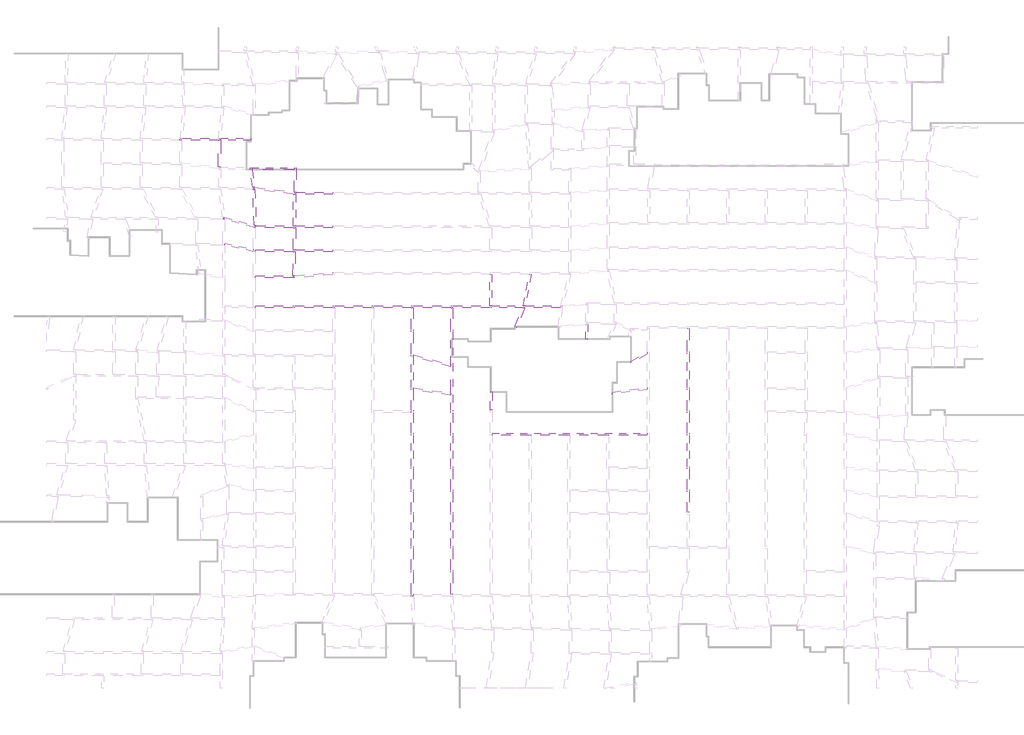
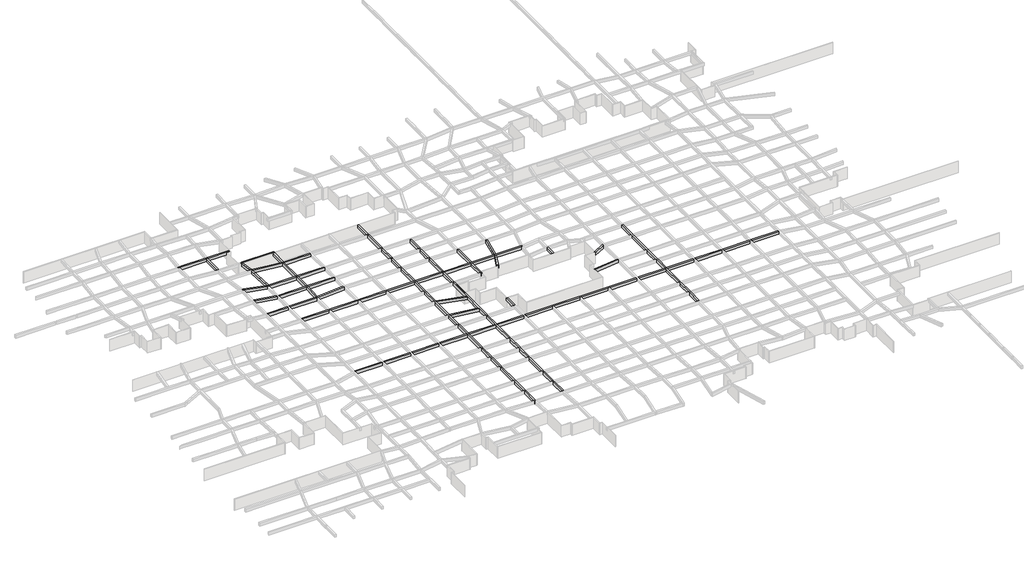
# One storey, part 28 of 45: 32 beams.
"""IFC4 building model written with IfcOpenShell, lengths in millimetres."""

import ifcopenshell
import ifcopenshell.guid

model = None  # the IFC model being written
_history = None  # IfcOwnerHistory: only IFC2X3 demands one
_inside = {}  # id of a spatial element -> (the spatial element, [elements in it])
_under = {}  # id of a project, library or spatial element -> (it, [spatial elements below it])
_declared = {}  # id of a project -> (the project, [libraries it declares])
_typed = {}  # id of a type object -> (the type object, [elements of that type])
_made_of = {}  # id of a material, layer set ... -> (it, [elements and type objects made of it])


def new_model(schema):
    """Start an empty IFC model of exactly this schema.

    Asked for "IFC4X3", IfcOpenShell would pick the latest addendum, in which some entities
    have other attributes; the version numbers below select the first issue.
    IFC2X3 requires an IfcOwnerHistory on every rooted entity: one is made here for all.
    """
    global model, _history
    if schema == "IFC4X3":
        model = ifcopenshell.file(schema_version=(4, 3, 0, 0))
    else:
        model = ifcopenshell.file(schema=schema)
    _inside.clear()
    _under.clear()
    _declared.clear()
    _typed.clear()
    _made_of.clear()
    _history = None
    if model.schema == "IFC2X3":
        org = make("IfcOrganization", Name="unknown")
        user = make(
            "IfcPersonAndOrganization",
            ThePerson=make("IfcPerson", FamilyName="unknown"),
            TheOrganization=org,
        )
        app = make(
            "IfcApplication",
            ApplicationDeveloper=org,
            Version="unknown",
            ApplicationFullName="unknown",
            ApplicationIdentifier="unknown",
        )
        _history = make(
            "IfcOwnerHistory",
            OwningUser=user,
            OwningApplication=app,
            ChangeAction="ADDED",
            CreationDate=0,
        )
    return model


def make(cls, **values):
    """One entity of the class cls with the attributes given. An attribute that is None is left unset."""
    return model.create_entity(
        cls, **{name: value for name, value in values.items() if value is not None}
    )


def rooted(cls, **values):
    """An entity with a GlobalId (a new one), such as an element, a storey or a relation."""
    return make(cls, GlobalId=ifcopenshell.guid.new(), OwnerHistory=_history, **values)


def si_unit(unit_type, name, prefix=None):
    """IfcSIUnit, for example si_unit("LENGTHUNIT", "METRE", prefix="MILLI")."""
    return make("IfcSIUnit", UnitType=unit_type, Prefix=prefix, Name=name)


def assignment(units):
    """IfcUnitAssignment: the units of a project."""
    return None if units is None else make("IfcUnitAssignment", Units=units)


def point(xyz):
    """IfcCartesianPoint."""
    return None if xyz is None else make("IfcCartesianPoint", Coordinates=xyz)


def direction(xyz):
    """IfcDirection."""
    return None if xyz is None else make("IfcDirection", DirectionRatios=xyz)


def frame(location, z_axis=None, x_axis=None):
    """IfcAxis2Placement3D, a coordinate frame: its origin and axes. An axis left out is left unset."""
    return make(
        "IfcAxis2Placement3D",
        Location=point(location),
        Axis=direction(z_axis),
        RefDirection=direction(x_axis),
    )


def origin():
    """The frame at (0, 0, 0) with its axes left unset."""
    return frame((0.0, 0.0, 0.0))


def place(relative_to, where):
    """IfcLocalPlacement: puts the frame where relative to a parent placement (None: the world)."""
    return make(
        "IfcLocalPlacement", PlacementRelTo=relative_to, RelativePlacement=where
    )


def context(
    kind, dimensions, precision=None, world=None, true_north=None, identifier=None
):
    """IfcGeometricRepresentationContext, for example the 3D "Model" context."""
    return make(
        "IfcGeometricRepresentationContext",
        ContextIdentifier=identifier,
        ContextType=kind,
        CoordinateSpaceDimension=dimensions,
        Precision=precision,
        WorldCoordinateSystem=world,
        TrueNorth=true_north,
    )


def project(units=None, contexts=None):
    """IfcProject with its units and contexts."""
    return rooted(
        "IfcProject",
        Name="project",
        RepresentationContexts=contexts,
        UnitsInContext=assignment(units),
    )


def spatial(cls, under=None, at=None, **own):
    """A site, building, storey or space (cls), placed at a placement, below another one or the project."""
    s = rooted(cls, ObjectPlacement=at, **own)
    if under is not None:
        _under.setdefault(under.id(), (under, []))[1].append(s)
    return s


def polyline(points):
    """IfcPolyline through the points."""
    return make("IfcPolyline", Points=[point(p) for p in points])


def outline(outer, holes=None, kind="AREA"):
    """IfcArbitraryClosedProfileDef: a profile drawn as a closed curve; with holes, ...WithVoids."""
    if holes is None:
        return make("IfcArbitraryClosedProfileDef", ProfileType=kind, OuterCurve=outer)
    return make(
        "IfcArbitraryProfileDefWithVoids",
        ProfileType=kind,
        OuterCurve=outer,
        InnerCurves=holes,
    )


def extrude(swept, where, along, depth):
    """IfcExtrudedAreaSolid: the profile swept, set in the frame where, extruded along a direction by depth."""
    return make(
        "IfcExtrudedAreaSolid",
        SweptArea=swept,
        Position=where,
        ExtrudedDirection=direction(along),
        Depth=depth,
    )


def faces_of(points, faces, orient=None, outer=None):
    """IfcFace entities. A face is a list of loops; a loop is a list of indices into points, from 0.

    orient and outer hold one flag for each loop. By default every Orientation is true, the
    first loop of a face is its IfcFaceOuterBound and the others are IfcFaceBound.
    """
    made = []
    for i, loops in enumerate(faces):
        bounds = []
        for j, loop in enumerate(loops):
            is_outer = j == 0 if outer is None else outer[i][j]
            bounds.append(
                make(
                    "IfcFaceOuterBound" if is_outer else "IfcFaceBound",
                    Bound=make("IfcPolyLoop", Polygon=[points[k] for k in loop]),
                    Orientation=True if orient is None else orient[i][j],
                )
            )
        made.append(make("IfcFace", Bounds=bounds))
    return made


def faceted_brep(points, faces, orient=None, outer=None, voids=None):
    """IfcFacetedBrep: a solid bounded by flat faces; with voids (closed shells), ...WithVoids."""
    shared = [point(p) for p in points]
    hull = make("IfcClosedShell", CfsFaces=faces_of(shared, faces, orient, outer))
    if voids is None:
        return make("IfcFacetedBrep", Outer=hull)
    return make(
        "IfcFacetedBrepWithVoids",
        Outer=hull,
        Voids=[
            make(cls, CfsFaces=faces_of(shared, fs, o, b)) for cls, fs, o, b in voids
        ],
    )


def shape(context_of_items, identifier, shape_type, items):
    """IfcShapeRepresentation: the items that make up one representation, for example the "Body"."""
    return make(
        "IfcShapeRepresentation",
        ContextOfItems=context_of_items,
        RepresentationIdentifier=identifier,
        RepresentationType=shape_type,
        Items=items,
    )


def made_of(thing, what):
    """Note that an element or type object is made of a material, layer set ...; save() writes the relation."""
    if what is not None:
        _made_of.setdefault(what.id(), (what, []))[1].append(thing)
    return thing


def element(
    cls,
    number,
    at=None,
    inside=None,
    cuts=None,
    type_object=None,
    material=None,
    context=None,
    identifier="Body",
    shape_type=None,
    held_by="IfcProductDefinitionShape",
    body=None,
    shapes=None,
    **own,
):
    """One element of the class cls, such as IfcWall. Its Tag is "e" and its number.

    at: its placement. inside: the storey or other place that contains it. cuts: it is an
    opening in that element (IfcRelVoidsElement). A single representation is given by context,
    identifier, shape_type and body (its items); several are given by shapes. held_by: the class
    of the entity that holds the representations. save() writes the other relations.
    """
    e = rooted(cls, Tag="e%d" % number, ObjectPlacement=at, **own)
    if body is not None:
        shapes = [shape(context, identifier, shape_type, body)]
    if shapes is not None:
        e.Representation = make(held_by, Representations=shapes)
    if inside is not None:
        _inside.setdefault(inside.id(), (inside, []))[1].append(e)
    if cuts is not None:
        rooted(
            "IfcRelVoidsElement", RelatingBuildingElement=cuts, RelatedOpeningElement=e
        )
    if type_object is not None:
        _typed.setdefault(type_object.id(), (type_object, []))[1].append(e)
    return made_of(e, material)


def aggregate(whole, parts):
    """IfcRelAggregates: a whole, such as a stair, and the parts it consists of."""
    return rooted("IfcRelAggregates", RelatingObject=whole, RelatedObjects=parts)


def save(model, path):
    """Write the relations noted so far, then the file.

    IfcRelAggregates (storeys below a building ...), IfcRelContainedInSpatialStructure (elements
    in a storey), IfcRelDefinesByType, IfcRelAssociatesMaterial and IfcRelDeclares: one each for
    every whole, place, type object, material and project.
    """
    for whole, parts in _under.values():
        aggregate(whole, parts)
    for where, things in _inside.values():
        rooted(
            "IfcRelContainedInSpatialStructure",
            RelatedElements=things,
            RelatingStructure=where,
        )
    for kind, things in _typed.values():
        rooted("IfcRelDefinesByType", RelatedObjects=things, RelatingType=kind)
    for what, things in _made_of.values():
        rooted("IfcRelAssociatesMaterial", RelatedObjects=things, RelatingMaterial=what)
    for by, libraries in _declared.values():
        rooted("IfcRelDeclares", RelatingContext=by, RelatedDefinitions=libraries)
    model.write(path)


model = new_model("IFC4")

# Units and contexts
model_context = context("Model", 3, world=origin())
ifc_project = project(units=[si_unit("LENGTHUNIT", "METRE", prefix="MILLI")], contexts=[model_context])

# Site, building, storey
site = spatial("IfcSite", under=ifc_project)
building = spatial("IfcBuilding", under=site)
storey = spatial("IfcBuildingStorey", under=building, Name="户型图", Elevation=0.0)

# Beams
placement = place(None, origin())
element("IfcBeam", 1, ObjectType="混凝土 - 矩形梁 : KL_beam", at=placement, inside=storey, context=model_context, shape_type="Brep", body=[
    faceted_brep([(-31589.1083091, 27984.5858537, 3300.0), (-31613.4317995, 28384.5858537, 3300.0), (-31838.0772004, 28384.5858537, 3300.0), (-38821.0090247, 28384.5858537, 3300.0), (-39228.4957027, 28384.5858537, 3300.0), (-45471.0209029, 28384.5858537, 3300.0), (-45871.0209029, 28384.5858537, 3300.0), (-53171.0209029, 28384.5858537, 3300.0), (-53571.0209029, 28384.5858537, 3300.0), (-60985.2176693, 28384.5858537, 3300.0), (-61385.2176693, 28384.5858537, 3300.0), (-68859.410716, 28384.5858537, 3300.0), (-69259.410716, 28384.5858537, 3300.0), (-76574.0592951, 28384.5858537, 3300.0), (-76974.0592951, 28384.5858537, 3300.0), (-84543.4535378, 28384.5858537, 3300.0), (-84943.4535378, 28384.5858537, 3300.0), (-92355.449792, 28384.5858537, 3300.0), (-92355.449792, 27984.5858537, 3300.0), (-84943.4535378, 27984.5858537, 3300.0), (-84543.4535378, 27984.5858537, 3300.0), (-76974.0592951, 27984.5858537, 3300.0), (-76574.0592951, 27984.5858537, 3300.0), (-69259.410716, 27984.5858537, 3300.0), (-68859.410716, 27984.5858537, 3300.0), (-61385.2176693, 27984.5858537, 3300.0), (-60985.2176693, 27984.5858537, 3300.0), (-53571.0209029, 27984.5858537, 3300.0), (-53171.0209029, 27984.5858537, 3300.0), (-45871.0209029, 27984.5858537, 3300.0), (-45471.0209029, 27984.5858537, 3300.0), (-39360.1406192, 27984.5858537, 3300.0), (-38928.7267221, 27984.5858537, 3300.0), (-31901.6167168, 27984.5858537, 3300.0), (-31613.4317995, 28384.5858537, 2500.0), (-31838.0772004, 28384.5858537, 2500.0), (-38821.0090247, 28384.5858537, 2500.0), (-39228.4957027, 28384.5858537, 2500.0), (-45471.0209029, 28384.5858537, 2500.0), (-45871.0209029, 28384.5858537, 2500.0), (-53171.0209029, 28384.5858537, 2500.0), (-53571.0209029, 28384.5858537, 2500.0), (-60985.2176693, 28384.5858537, 2500.0), (-61385.2176693, 28384.5858537, 2500.0), (-68859.410716, 28384.5858537, 2500.0), (-69259.410716, 28384.5858537, 2500.0), (-76574.0592951, 28384.5858537, 2500.0), (-76974.0592951, 28384.5858537, 2500.0), (-84543.4535378, 28384.5858537, 2500.0), (-84943.4535378, 28384.5858537, 2500.0), (-92355.449792, 28384.5858537, 2500.0), (-31589.1083091, 27984.5858537, 2500.0), (-31901.6167168, 27984.5858537, 2500.0), (-38928.7267221, 27984.5858537, 2500.0), (-39360.1406192, 27984.5858537, 2500.0), (-45471.0209029, 27984.5858537, 2500.0), (-45871.0209029, 27984.5858537, 2500.0), (-53171.0209029, 27984.5858537, 2500.0), (-53571.0209029, 27984.5858537, 2500.0), (-60985.2176693, 27984.5858537, 2500.0), (-61385.2176693, 27984.5858537, 2500.0), (-68859.410716, 27984.5858537, 2500.0), (-69259.410716, 27984.5858537, 2500.0), (-76574.0592951, 27984.5858537, 2500.0), (-76974.0592951, 27984.5858537, 2500.0), (-84543.4535378, 27984.5858537, 2500.0), (-84943.4535378, 27984.5858537, 2500.0), (-92355.449792, 27984.5858537, 2500.0)], [[[0, 1, 2, 3, 4, 5, 6, 7, 8, 9, 10, 11, 12, 13, 14, 15, 16, 17, 18, 19, 20, 21, 22, 23, 24, 25, 26, 27, 28, 29, 30, 31, 32, 33]], [[1, 34, 35, 36, 37, 38, 39, 40, 41, 42, 43, 44, 45, 46, 47, 48, 49, 50, 17, 16, 15, 14, 13, 12, 11, 10, 9, 8, 7, 6, 5, 4, 3, 2]], [[34, 51, 52, 53, 54, 55, 56, 57, 58, 59, 60, 61, 62, 63, 64, 65, 66, 67, 50, 49, 48, 47, 46, 45, 44, 43, 42, 41, 40, 39, 38, 37, 36, 35]], [[51, 0, 33, 32, 31, 30, 29, 28, 27, 26, 25, 24, 23, 22, 21, 20, 19, 18, 67, 66, 65, 64, 63, 62, 61, 60, 59, 58, 57, 56, 55, 54, 53, 52]], [[0, 51, 34, 1]], [[18, 17, 50, 67]]]),
])
element("IfcBeam", 2, ObjectType="混凝土 - 矩形梁 : KL_beam", at=placement, inside=storey, context=model_context, shape_type="Brep", body=[
    faceted_brep([(-60985.2176693, 55433.7567637, 3300.0), (-60985.2176693, 55433.7567637, 2500.0), (-61385.2176693, 55433.7567637, 2500.0), (-61385.2176693, 55433.7567637, 3300.0), (-60985.2176693, 50850.070339, 3300.0), (-61385.2176693, 50850.070339, 3300.0), (-61385.2176693, 50850.070339, 2500.0), (-60985.2176693, 50850.070339, 2500.0)], [[[0, 1, 2, 3]], [[4, 5, 6, 7]], [[0, 3, 5, 4]], [[3, 2, 6, 5]], [[2, 1, 7, 6]], [[1, 0, 4, 7]]]),
    faceted_brep([(-60985.2176693, -29259.522509, 3300.0), (-60985.2176693, -28866.2296815, 3300.0), (-60985.2176693, -24466.2432363, 3300.0), (-60985.2176693, -24066.2432363, 3300.0), (-60985.2176693, -19666.2432363, 3300.0), (-60985.2176693, -19266.2432363, 3300.0), (-60985.2176693, -13006.533538, 3300.0), (-60985.2176693, -12606.533538, 3300.0), (-60985.2176693, -8506.533538, 3300.0), (-60985.2176693, -8106.533538, 3300.0), (-60985.2176693, -3951.5199121, 3300.0), (-60985.2176693, -3551.5199121, 3300.0), (-60985.2176693, 2719.5822838, 3300.0), (-60985.2176693, 3119.5822838, 3300.0), (-60985.2176693, 7200.318112, 3300.0), (-60985.2176693, 7600.318112, 3300.0), (-60985.2176693, 11670.0801126, 3300.0), (-60985.2176693, 12074.0111416, 3300.0), (-60985.2176693, 18259.8013996, 3300.0), (-60985.2176693, 18673.9118717, 3300.0), (-60985.2176693, 23171.3370449, 3300.0), (-60985.2176693, 23571.3370449, 3300.0), (-60985.2176693, 27984.5858537, 3300.0), (-61385.2176693, 27984.5858537, 3300.0), (-61385.2176693, 23571.3370449, 3300.0), (-61385.2176693, 23171.3370449, 3300.0), (-61385.2176693, 18720.4464741, 3300.0), (-61385.2176693, 18320.4464741, 3300.0), (-61385.2176693, 12100.217385, 3300.0), (-61385.2176693, 11700.217385, 3300.0), (-61385.2176693, 7600.318112, 3300.0), (-61385.2176693, 7200.318112, 3300.0), (-61385.2176693, 3119.5822838, 3300.0), (-61385.2176693, 2719.5822838, 3300.0), (-61385.2176693, -3551.5199121, 3300.0), (-61385.2176693, -3951.5199121, 3300.0), (-61385.2176693, -8106.533538, 3300.0), (-61385.2176693, -8506.533538, 3300.0), (-61385.2176693, -12606.533538, 3300.0), (-61385.2176693, -13006.533538, 3300.0), (-61385.2176693, -19266.2432363, 3300.0), (-61385.2176693, -19666.2432363, 3300.0), (-61385.2176693, -24066.2432363, 3300.0), (-61385.2176693, -24466.2432363, 3300.0), (-61385.2176693, -28859.2888151, 3300.0), (-61385.2176693, -29259.522509, 3300.0), (-61385.2176693, 27984.5858537, 2500.0), (-61385.2176693, 23571.3370449, 2500.0), (-61385.2176693, 23171.3370449, 2500.0), (-61385.2176693, 18720.4464741, 2500.0), (-61385.2176693, 18320.4464741, 2500.0), (-61385.2176693, 12100.217385, 2500.0), (-61385.2176693, 11700.217385, 2500.0), (-61385.2176693, 7600.318112, 2500.0), (-61385.2176693, 7200.318112, 2500.0), (-61385.2176693, 3119.5822838, 2500.0), (-61385.2176693, 2719.5822838, 2500.0), (-61385.2176693, -3551.5199121, 2500.0), (-61385.2176693, -3951.5199121, 2500.0), (-61385.2176693, -8106.533538, 2500.0), (-61385.2176693, -8506.533538, 2500.0), (-61385.2176693, -12606.533538, 2500.0), (-61385.2176693, -13006.533538, 2500.0), (-61385.2176693, -19266.2432363, 2500.0), (-61385.2176693, -19666.2432363, 2500.0), (-61385.2176693, -24066.2432363, 2500.0), (-61385.2176693, -24466.2432363, 2500.0), (-61385.2176693, -28859.2888151, 2500.0), (-61385.2176693, -29259.522509, 2500.0), (-60985.2176693, 27984.5858537, 2500.0), (-60985.2176693, 23571.3370449, 2500.0), (-60985.2176693, 23171.3370449, 2500.0), (-60985.2176693, 18673.9118717, 2500.0), (-60985.2176693, 18259.8013996, 2500.0), (-60985.2176693, 12074.0111416, 2500.0), (-60985.2176693, 11670.0801126, 2500.0), (-60985.2176693, 7600.318112, 2500.0), (-60985.2176693, 7200.318112, 2500.0), (-60985.2176693, 3119.5822838, 2500.0), (-60985.2176693, 2719.5822838, 2500.0), (-60985.2176693, -3551.5199121, 2500.0), (-60985.2176693, -3951.5199121, 2500.0), (-60985.2176693, -8106.533538, 2500.0), (-60985.2176693, -8506.533538, 2500.0), (-60985.2176693, -12606.533538, 2500.0), (-60985.2176693, -13006.533538, 2500.0), (-60985.2176693, -19266.2432363, 2500.0), (-60985.2176693, -19666.2432363, 2500.0), (-60985.2176693, -24066.2432363, 2500.0), (-60985.2176693, -24466.2432363, 2500.0), (-60985.2176693, -28866.2296815, 2500.0), (-60985.2176693, -29259.522509, 2500.0)], [[[0, 1, 2, 3, 4, 5, 6, 7, 8, 9, 10, 11, 12, 13, 14, 15, 16, 17, 18, 19, 20, 21, 22, 23, 24, 25, 26, 27, 28, 29, 30, 31, 32, 33, 34, 35, 36, 37, 38, 39, 40, 41, 42, 43, 44, 45]], [[45, 44, 43, 42, 41, 40, 39, 38, 37, 36, 35, 34, 33, 32, 31, 30, 29, 28, 27, 26, 25, 24, 23, 46, 47, 48, 49, 50, 51, 52, 53, 54, 55, 56, 57, 58, 59, 60, 61, 62, 63, 64, 65, 66, 67, 68]], [[68, 67, 66, 65, 64, 63, 62, 61, 60, 59, 58, 57, 56, 55, 54, 53, 52, 51, 50, 49, 48, 47, 46, 69, 70, 71, 72, 73, 74, 75, 76, 77, 78, 79, 80, 81, 82, 83, 84, 85, 86, 87, 88, 89, 90, 91]], [[22, 21, 20, 19, 18, 17, 16, 15, 14, 13, 12, 11, 10, 9, 8, 7, 6, 5, 4, 3, 2, 1, 0, 91, 90, 89, 88, 87, 86, 85, 84, 83, 82, 81, 80, 79, 78, 77, 76, 75, 74, 73, 72, 71, 70, 69]], [[23, 22, 69, 46]], [[0, 45, 68, 91]]]),
    faceted_brep([(-60985.2176693, 28384.5858537, 3300.0), (-61385.2176693, 28384.5858537, 3300.0), (-61385.2176693, 28384.5858537, 2500.0), (-60985.2176693, 28384.5858537, 2500.0), (-60985.2176693, 34571.3370449, 3300.0), (-61385.2176693, 34571.3370449, 3300.0), (-61385.2176693, 34571.3370449, 2500.0), (-60985.2176693, 34571.3370449, 2500.0)], [[[0, 1, 2, 3]], [[1, 0, 4, 5]], [[2, 1, 5, 6]], [[3, 2, 6, 7]], [[0, 3, 7, 4]], [[5, 4, 7, 6]]]),
    faceted_brep([(-60985.2176693, 34971.3370449, 3300.0), (-61385.2176693, 34971.3370449, 3300.0), (-61385.2176693, 34971.3370449, 2500.0), (-60985.2176693, 34971.3370449, 2500.0), (-60985.2176693, 39070.5101546, 3300.0), (-61385.2176693, 39070.5101546, 3300.0), (-61385.2176693, 39070.5101546, 2500.0), (-60985.2176693, 39070.5101546, 2500.0)], [[[0, 1, 2, 3]], [[1, 0, 4, 5]], [[2, 1, 5, 6]], [[3, 2, 6, 7]], [[0, 3, 7, 4]], [[5, 4, 7, 6]]]),
    faceted_brep([(-60985.2176693, 39470.5101546, 3300.0), (-61385.2176693, 39470.5101546, 3300.0), (-61385.2176693, 39470.5101546, 2500.0), (-60985.2176693, 39470.5101546, 2500.0), (-60985.2176693, 43842.2010773, 3300.0), (-61385.2176693, 43842.2010773, 3300.0), (-61385.2176693, 43842.2010773, 2500.0), (-60985.2176693, 43842.2010773, 2500.0)], [[[0, 1, 2, 3]], [[1, 0, 4, 5]], [[2, 1, 5, 6]], [[3, 2, 6, 7]], [[0, 3, 7, 4]], [[5, 4, 7, 6]]]),
    faceted_brep([(-60985.2176693, 44242.2010773, 3300.0), (-61385.2176693, 44242.2010773, 3300.0), (-61385.2176693, 44242.2010773, 2500.0), (-60985.2176693, 44242.2010773, 2500.0), (-60985.2176693, 50450.070339, 3300.0), (-61385.2176693, 50450.070339, 3300.0), (-61385.2176693, 50450.070339, 2500.0), (-60985.2176693, 50450.070339, 2500.0)], [[[0, 1, 2, 3]], [[1, 0, 4, 5]], [[2, 1, 5, 6]], [[3, 2, 6, 7]], [[0, 3, 7, 4]], [[5, 4, 7, 6]]]),
])
element("IfcBeam", 3, ObjectType="混凝土 - 矩形梁 : KL_beam", at=placement, inside=storey, context=model_context, shape_type="Brep", body=[
    faceted_brep([(-53171.0209029, 43842.2010773, 3300.0), (-53571.0209029, 43842.2010773, 3300.0), (-53571.0209029, 39470.5101546, 3300.0), (-53171.0209029, 39470.5101546, 3300.0), (-53571.0209029, 43842.2010773, 2500.0), (-53571.0209029, 39470.5101546, 2500.0), (-53171.0209029, 43842.2010773, 2500.0), (-53171.0209029, 39470.5101546, 2500.0)], [[[0, 1, 2, 3]], [[1, 4, 5, 2]], [[4, 6, 7, 5]], [[6, 0, 3, 7]], [[1, 0, 6, 4]], [[3, 2, 5, 7]]]),
    faceted_brep([(-53171.0209029, 28384.5858537, 3300.0), (-53571.0209029, 28384.5858537, 3300.0), (-53571.0209029, 28384.5858537, 2500.0), (-53171.0209029, 28384.5858537, 2500.0), (-53571.0209029, 34571.3370449, 3300.0), (-53171.0209029, 34571.3370449, 3300.0), (-53171.0209029, 34571.3370449, 2500.0), (-53571.0209029, 34571.3370449, 2500.0)], [[[0, 1, 2, 3]], [[4, 5, 6, 7]], [[1, 0, 5, 4]], [[2, 1, 4, 7]], [[3, 2, 7, 6]], [[0, 3, 6, 5]]]),
    faceted_brep([(-53571.0209029, 27984.5858537, 3300.0), (-53171.0209029, 27984.5858537, 3300.0), (-53171.0209029, 27984.5858537, 2500.0), (-53571.0209029, 27984.5858537, 2500.0), (-53571.0209029, 23571.3370449, 3300.0), (-53571.0209029, 23171.3370449, 3300.0), (-53571.0209029, 16687.2838357, 3300.0), (-53571.0209029, 16273.1733635, 3300.0), (-53571.0209029, 11032.0137394, 3300.0), (-53571.0209029, 10628.0827104, 3300.0), (-53571.0209029, 7600.318112, 3300.0), (-53571.0209029, 7200.318112, 3300.0), (-53571.0209029, 3119.5822838, 3300.0), (-53571.0209029, 2719.5822838, 3300.0), (-53571.0209029, -3551.5199121, 3300.0), (-53571.0209029, -3951.5199121, 3300.0), (-53571.0209029, -8106.533538, 3300.0), (-53571.0209029, -8506.533538, 3300.0), (-53571.0209029, -12606.533538, 3300.0), (-53571.0209029, -13006.533538, 3300.0), (-53571.0209029, -19266.2432363, 3300.0), (-53571.0209029, -19666.2432363, 3300.0), (-53571.0209029, -24066.2432363, 3300.0), (-53571.0209029, -24466.2432363, 3300.0), (-53571.0209029, -28866.2296815, 3300.0), (-53171.0209029, -28866.2296815, 3300.0), (-53171.0209029, -24466.2432363, 3300.0), (-53171.0209029, -24066.2432363, 3300.0), (-53171.0209029, -19666.2432363, 3300.0), (-53171.0209029, -19266.2432363, 3300.0), (-53171.0209029, -13006.533538, 3300.0), (-53171.0209029, -12606.533538, 3300.0), (-53171.0209029, -8506.533538, 3300.0), (-53171.0209029, -8106.533538, 3300.0), (-53171.0209029, -3951.5199121, 3300.0), (-53171.0209029, -3551.5199121, 3300.0), (-53171.0209029, 2719.5822838, 3300.0), (-53171.0209029, 3119.5822838, 3300.0), (-53171.0209029, 7200.318112, 3300.0), (-53171.0209029, 7600.318112, 3300.0), (-53171.0209029, 23171.3370449, 3300.0), (-53171.0209029, 23571.3370449, 3300.0), (-53571.0209029, 23571.3370449, 2500.0), (-53571.0209029, 23171.3370449, 2500.0), (-53571.0209029, 16687.2838357, 2500.0), (-53571.0209029, 16273.1733635, 2500.0), (-53571.0209029, 11032.0137394, 2500.0), (-53571.0209029, 10628.0827104, 2500.0), (-53571.0209029, 7600.318112, 2500.0), (-53571.0209029, 7200.318112, 2500.0), (-53571.0209029, 3119.5822838, 2500.0), (-53571.0209029, 2719.5822838, 2500.0), (-53571.0209029, -3551.5199121, 2500.0), (-53571.0209029, -3951.5199121, 2500.0), (-53571.0209029, -8106.533538, 2500.0), (-53571.0209029, -8506.533538, 2500.0), (-53571.0209029, -12606.533538, 2500.0), (-53571.0209029, -13006.533538, 2500.0), (-53571.0209029, -19266.2432363, 2500.0), (-53571.0209029, -19666.2432363, 2500.0), (-53571.0209029, -24066.2432363, 2500.0), (-53571.0209029, -24466.2432363, 2500.0), (-53571.0209029, -28866.2296815, 2500.0), (-53171.0209029, 23571.3370449, 2500.0), (-53171.0209029, 23171.3370449, 2500.0), (-53171.0209029, 7600.318112, 2500.0), (-53171.0209029, 7200.318112, 2500.0), (-53171.0209029, 3119.5822838, 2500.0), (-53171.0209029, 2719.5822838, 2500.0), (-53171.0209029, -3551.5199121, 2500.0), (-53171.0209029, -3951.5199121, 2500.0), (-53171.0209029, -8106.533538, 2500.0), (-53171.0209029, -8506.533538, 2500.0), (-53171.0209029, -12606.533538, 2500.0), (-53171.0209029, -13006.533538, 2500.0), (-53171.0209029, -19266.2432363, 2500.0), (-53171.0209029, -19666.2432363, 2500.0), (-53171.0209029, -24066.2432363, 2500.0), (-53171.0209029, -24466.2432363, 2500.0), (-53171.0209029, -28866.2296815, 2500.0)], [[[0, 1, 2, 3]], [[1, 0, 4, 5, 6, 7, 8, 9, 10, 11, 12, 13, 14, 15, 16, 17, 18, 19, 20, 21, 22, 23, 24, 25, 26, 27, 28, 29, 30, 31, 32, 33, 34, 35, 36, 37, 38, 39, 40, 41]], [[0, 3, 42, 43, 44, 45, 46, 47, 48, 49, 50, 51, 52, 53, 54, 55, 56, 57, 58, 59, 60, 61, 62, 24, 23, 22, 21, 20, 19, 18, 17, 16, 15, 14, 13, 12, 11, 10, 9, 8, 7, 6, 5, 4]], [[3, 2, 63, 64, 65, 66, 67, 68, 69, 70, 71, 72, 73, 74, 75, 76, 77, 78, 79, 62, 61, 60, 59, 58, 57, 56, 55, 54, 53, 52, 51, 50, 49, 48, 47, 46, 45, 44, 43, 42]], [[2, 1, 41, 40, 39, 38, 37, 36, 35, 34, 33, 32, 31, 30, 29, 28, 27, 26, 25, 79, 78, 77, 76, 75, 74, 73, 72, 71, 70, 69, 68, 67, 66, 65, 64, 63]], [[25, 24, 62, 79]]]),
    faceted_brep([(-53171.0209029, 34971.3370449, 3300.0), (-53571.0209029, 34971.3370449, 3300.0), (-53571.0209029, 34971.3370449, 2500.0), (-53171.0209029, 34971.3370449, 2500.0), (-53571.0209029, 39070.5101546, 3300.0), (-53171.0209029, 39070.5101546, 3300.0), (-53171.0209029, 39070.5101546, 2500.0), (-53571.0209029, 39070.5101546, 2500.0)], [[[0, 1, 2, 3]], [[4, 5, 6, 7]], [[1, 0, 5, 4]], [[2, 1, 4, 7]], [[3, 2, 7, 6]], [[0, 3, 6, 5]]]),
])
element("IfcBeam", 4, ObjectType="混凝土 - 矩形梁 : KL_beam", at=placement, inside=storey, context=model_context, shape_type="Brep", body=[
    faceted_brep([(-6328.2347705, 23868.127427, 3300.0), (-6728.2347705, 23868.127427, 3300.0), (-6728.2347705, 19231.9876735, 3300.0), (-6728.2347705, 18831.9876735, 3300.0), (-6728.2347705, 12131.9876735, 3300.0), (-6728.2347705, 11731.9876735, 3300.0), (-6728.2347705, 7519.5822838, 3300.0), (-6728.2347705, 7119.5822838, 3300.0), (-6728.2347705, 3119.5822838, 3300.0), (-6728.2347705, 2719.5822838, 3300.0), (-6728.2347705, -3551.5199121, 3300.0), (-6728.2347705, -3951.5199121, 3300.0), (-6728.2347705, -8106.533538, 3300.0), (-6728.2347705, -8506.533538, 3300.0), (-6728.2347705, -12606.533538, 3300.0), (-6328.2347705, -12606.533538, 3300.0), (-6328.2347705, -8506.533538, 3300.0), (-6328.2347705, -8106.533538, 3300.0), (-6328.2347705, -3951.5199121, 3300.0), (-6328.2347705, -3551.5199121, 3300.0), (-6328.2347705, 2719.5822838, 3300.0), (-6328.2347705, 3119.5822838, 3300.0), (-6328.2347705, 7119.5822838, 3300.0), (-6328.2347705, 7519.5822838, 3300.0), (-6328.2347705, 11731.9876735, 3300.0), (-6328.2347705, 12131.9876735, 3300.0), (-6328.2347705, 18831.9876735, 3300.0), (-6328.2347705, 19231.9876735, 3300.0), (-6728.2347705, 23868.127427, 2500.0), (-6728.2347705, 19231.9876735, 2500.0), (-6728.2347705, 18831.9876735, 2500.0), (-6728.2347705, 12131.9876735, 2500.0), (-6728.2347705, 11731.9876735, 2500.0), (-6728.2347705, 7519.5822838, 2500.0), (-6728.2347705, 7119.5822838, 2500.0), (-6728.2347705, 3119.5822838, 2500.0), (-6728.2347705, 2719.5822838, 2500.0), (-6728.2347705, -3551.5199121, 2500.0), (-6728.2347705, -3951.5199121, 2500.0), (-6728.2347705, -8106.533538, 2500.0), (-6728.2347705, -8506.533538, 2500.0), (-6728.2347705, -12606.533538, 2500.0), (-6328.2347705, 23868.127427, 2500.0), (-6328.2347705, 19231.9876735, 2500.0), (-6328.2347705, 18831.9876735, 2500.0), (-6328.2347705, 12131.9876735, 2500.0), (-6328.2347705, 11731.9876735, 2500.0), (-6328.2347705, 7519.5822838, 2500.0), (-6328.2347705, 7119.5822838, 2500.0), (-6328.2347705, 3119.5822838, 2500.0), (-6328.2347705, 2719.5822838, 2500.0), (-6328.2347705, -3551.5199121, 2500.0), (-6328.2347705, -3951.5199121, 2500.0), (-6328.2347705, -8106.533538, 2500.0), (-6328.2347705, -8506.533538, 2500.0), (-6328.2347705, -12606.533538, 2500.0)], [[[0, 1, 2, 3, 4, 5, 6, 7, 8, 9, 10, 11, 12, 13, 14, 15, 16, 17, 18, 19, 20, 21, 22, 23, 24, 25, 26, 27]], [[1, 28, 29, 30, 31, 32, 33, 34, 35, 36, 37, 38, 39, 40, 41, 14, 13, 12, 11, 10, 9, 8, 7, 6, 5, 4, 3, 2]], [[28, 42, 43, 44, 45, 46, 47, 48, 49, 50, 51, 52, 53, 54, 55, 41, 40, 39, 38, 37, 36, 35, 34, 33, 32, 31, 30, 29]], [[42, 0, 27, 26, 25, 24, 23, 22, 21, 20, 19, 18, 17, 16, 15, 55, 54, 53, 52, 51, 50, 49, 48, 47, 46, 45, 44, 43]], [[1, 0, 42, 28]], [[15, 14, 41, 55]]]),
])
element("IfcBeam", 5, ObjectType="混凝土 - 矩形梁 : KL_beam", at=placement, inside=storey, context=model_context, shape_type="SweptSolid", body=[
    extrude(outline(polyline([(-38821.0090247, 28384.5858537), (-39228.4957027, 28384.5858537), (-38025.9130936, 34571.3370449), (-37618.4264156, 34571.3370449), (-38821.0090247, 28384.5858537)])), frame((0.0, 0.0, 2500.0), z_axis=(0.0, 0.0, 1.0), x_axis=(1.0, 0.0, 0.0)), (0.0, 0.0, 1.0), 800.0),
])
element("IfcBeam", 6, ObjectType="混凝土 - 矩形梁 : KL_beam", at=placement, inside=storey, context=model_context, shape_type="Brep", body=[
    faceted_brep([(-45471.0209029, 34571.3370449, 3300.0), (-45871.0209029, 34571.3370449, 3300.0), (-45871.0209029, 28384.5858537, 3300.0), (-45471.0209029, 28384.5858537, 3300.0), (-45871.0209029, 34571.3370449, 2500.0), (-45871.0209029, 28384.5858537, 2500.0), (-45471.0209029, 34571.3370449, 2500.0), (-45471.0209029, 28384.5858537, 2500.0)], [[[0, 1, 2, 3]], [[1, 4, 5, 2]], [[4, 6, 7, 5]], [[6, 0, 3, 7]], [[1, 0, 6, 4]], [[3, 2, 5, 7]]]),
    faceted_brep([(-45871.0209029, 27984.5858537, 3300.0), (-45471.0209029, 27984.5858537, 3300.0), (-45471.0209029, 27984.5858537, 2500.0), (-45871.0209029, 27984.5858537, 2500.0), (-45871.0209029, 23171.3370449, 3300.0), (-45471.0209029, 23171.3370449, 3300.0), (-45871.0209029, 23571.3370449, 3300.0), (-45871.0209029, 23171.3370449, 2500.0), (-45871.0209029, 23571.3370449, 2500.0), (-45471.0209029, 23171.3370449, 2500.0)], [[[0, 1, 2, 3]], [[4, 5, 1, 0, 6]], [[7, 4, 6, 0, 3, 8]], [[9, 7, 8, 3, 2]], [[5, 9, 2, 1]], [[5, 4, 7, 9]]]),
])
element("IfcBeam", 7, ObjectType="混凝土 - 矩形梁 : KL_beam", at=placement, inside=storey, context=model_context, shape_type="Brep", body=[
    faceted_brep([(-99250.9559359, 61170.3096597, 3300.0), (-99209.2278595, 61570.3096597, 3300.0), (-99611.3985103, 61570.3096597, 3300.0), (-106787.9351309, 61570.3096597, 3300.0), (-107189.4630659, 61570.3096597, 3300.0), (-107354.1744669, 61570.3096597, 3300.0), (-107354.1744669, 61170.3096597, 3300.0), (-106954.1744669, 61170.3096597, 3300.0), (-99631.1820439, 61170.3096597, 3300.0), (-99250.9559359, 61170.3096597, 2500.0), (-107354.1744669, 61170.3096597, 2500.0), (-106954.1744669, 61170.3096597, 2500.0), (-99631.1820439, 61170.3096597, 2500.0), (-99209.2278595, 61570.3096597, 2500.0), (-107354.1744669, 61570.3096597, 2500.0), (-107189.4630659, 61570.3096597, 2500.0), (-106787.9351309, 61570.3096597, 2500.0), (-99611.3985103, 61570.3096597, 2500.0)], [[[0, 1, 2, 3, 4, 5, 6, 7, 8]], [[9, 0, 8, 7, 6, 10, 11, 12]], [[13, 9, 12, 11, 10, 14, 15, 16, 17]], [[1, 13, 17, 16, 15, 14, 5, 4, 3, 2]], [[1, 0, 9, 13]], [[6, 5, 14, 10]]]),
])
element("IfcBeam", 8, ObjectType="混凝土 - 矩形梁 : KL_beam", at=placement, inside=storey, context=model_context, shape_type="Brep", body=[
    faceted_brep([(-93231.1772231, 61570.3096597, 3300.0), (-93231.1772231, 61170.3096597, 3300.0), (-93231.1772231, 61170.3096597, 2500.0), (-93231.1772231, 61570.3096597, 2500.0), (-99209.2278595, 61570.3096597, 3300.0), (-99250.9559359, 61170.3096597, 3300.0), (-99231.1820439, 61170.3096597, 3300.0), (-99250.9559359, 61170.3096597, 2500.0), (-99231.1820439, 61170.3096597, 2500.0), (-99209.2278595, 61570.3096597, 2500.0)], [[[0, 1, 2, 3]], [[1, 0, 4, 5, 6]], [[2, 1, 6, 5, 7, 8]], [[3, 2, 8, 7, 9]], [[0, 3, 9, 4]], [[5, 4, 9, 7]]]),
])
element("IfcBeam", 9, ObjectType="混凝土 - 矩形梁 : KL_beam", at=placement, inside=storey, context=model_context, shape_type="Brep", body=[
    faceted_brep([(-84245.4455357, 50827.038832, 3300.0), (-84645.4455357, 50876.1526564, 3300.0), (-92452.2931975, 51834.7130186, 3300.0), (-92616.9469361, 51854.9299556, 3300.0), (-92641.4119842, 51454.9299556, 3300.0), (-92421.2676267, 51427.8996273, 3300.0), (-84764.7545436, 50487.7980304, 3300.0), (-84364.7545436, 50438.684206, 3300.0), (-84294.1932731, 50430.0203714, 3300.0), (-84289.9298602, 50464.7430833, 3300.0), (-92641.4119842, 51454.9299556, 2500.0), (-92421.2676267, 51427.8996273, 2500.0), (-84764.7545436, 50487.7980304, 2500.0), (-84364.7545436, 50438.684206, 2500.0), (-84294.1932731, 50430.0203714, 2500.0), (-92616.9469361, 51854.9299556, 2500.0), (-92452.2931975, 51834.7130186, 2500.0), (-84645.4455357, 50876.1526564, 2500.0), (-84245.4455357, 50827.038832, 2500.0), (-84289.9298602, 50464.7430833, 2500.0)], [[[0, 1, 2, 3, 4, 5, 6, 7, 8, 9]], [[8, 7, 6, 5, 4, 10, 11, 12, 13, 14]], [[14, 13, 12, 11, 10, 15, 16, 17, 18, 19]], [[3, 2, 1, 0, 18, 17, 16, 15]], [[3, 15, 10, 4]], [[0, 9, 8, 14, 19, 18]]]),
])
element("IfcBeam", 10, ObjectType="混凝土 - 矩形梁 : KL_beam", at=placement, inside=storey, context=model_context, shape_type="Brep", body=[
    faceted_brep([(-92452.2931975, 51834.7130186, 3300.0), (-92946.3477439, 55350.0937791, 3300.0), (-93002.5640778, 55750.0937791, 3300.0), (-93021.5786579, 55747.4214542, 3300.0), (-93398.6713053, 55694.4245387, 3300.0), (-93350.7020276, 55353.1053927, 3300.0), (-92859.0655317, 51854.9299556, 3300.0), (-92616.9469361, 51854.9299556, 3300.0), (-92452.2931975, 51834.7130186, 2500.0), (-92946.3477439, 55350.0937791, 2500.0), (-93002.5640778, 55750.0937791, 2500.0), (-92616.9469361, 51854.9299556, 2500.0), (-92859.0655317, 51854.9299556, 2500.0), (-93350.7020276, 55353.1053927, 2500.0), (-93398.6713053, 55694.4245387, 2500.0), (-93021.5786579, 55747.4214542, 2500.0)], [[[0, 1, 2, 3, 4, 5, 6, 7]], [[2, 1, 0, 8, 9, 10]], [[10, 9, 8, 11, 12, 13, 14, 15]], [[4, 14, 13, 12, 6, 5]], [[0, 7, 11, 8]], [[7, 6, 12, 11]], [[4, 3, 2, 10, 15, 14]]]),
])
element("IfcBeam", 11, ObjectType="混凝土 - 矩形梁 : KL_beam", at=placement, inside=storey, context=model_context, shape_type="Brep", body=[
    faceted_brep([(-84245.4455357, 55750.0937791, 3300.0), (-84645.4455357, 55750.0937791, 3300.0), (-84645.4455357, 55350.0937791, 3300.0), (-84645.4455357, 50876.1526564, 3300.0), (-84245.4455357, 50827.038832, 3300.0), (-84245.4455357, 50864.7430833, 3300.0), (-84245.4455357, 55750.0937791, 2500.0), (-84245.4455357, 50827.038832, 2500.0), (-84245.4455357, 50864.7430833, 2500.0), (-84645.4455357, 55750.0937791, 2500.0), (-84645.4455357, 50876.1526564, 2500.0), (-84645.4455357, 55350.0937791, 2500.0)], [[[0, 1, 2, 3, 4, 5]], [[6, 0, 5, 4, 7, 8]], [[9, 6, 8, 7, 10, 11]], [[1, 9, 11, 10, 3, 2]], [[4, 3, 10, 7]], [[1, 0, 6, 9]]]),
])
element("IfcBeam", 12, ObjectType="混凝土 - 矩形梁 : KL_beam", at=placement, inside=storey, context=model_context, shape_type="SweptSolid", body=[
    extrude(outline(polyline([(-92946.3477439, 55350.0937791), (-93002.5640778, 55750.0937791), (-84645.4455357, 55750.0937791), (-84645.4455357, 55350.0937791), (-92946.3477439, 55350.0937791)])), frame((0.0, 0.0, 2500.0), z_axis=(0.0, 0.0, 1.0), x_axis=(1.0, 0.0, 0.0)), (0.0, 0.0, 1.0), 800.0),
])
element("IfcBeam", 13, ObjectType="混凝土 - 矩形梁 : KL_beam", at=placement, inside=storey, context=model_context, shape_type="Brep", body=[
    faceted_brep([(-99631.1820439, 55886.0592094, 3300.0), (-99363.3334842, 55858.1171964, 3300.0), (-99231.1820439, 55855.8104845, 3300.0), (-99231.1820439, 61170.3096597, 3300.0), (-99250.9559359, 61170.3096597, 3300.0), (-99631.1820439, 61170.3096597, 3300.0), (-99631.1820439, 55886.0592094, 2500.0), (-99631.1820439, 61170.3096597, 2500.0), (-99363.3334842, 55858.1171964, 2500.0), (-99250.9559359, 61170.3096597, 2500.0), (-99231.1820439, 61170.3096597, 2500.0), (-99231.1820439, 55855.8104845, 2500.0)], [[[0, 1, 2, 3, 4, 5]], [[6, 0, 5, 7]], [[8, 6, 7, 9, 10, 11]], [[10, 3, 2, 11]], [[1, 0, 6, 8]], [[7, 5, 4, 3, 10, 9]], [[2, 1, 8, 11]]]),
])
element("IfcBeam", 14, ObjectType="混凝土 - 矩形梁 : KL_beam", at=placement, inside=storey, context=model_context, shape_type="Brep", body=[
    faceted_brep([(-92329.1192925, 44242.2010773, 3300.0), (-92564.8658583, 44305.3691792, 3300.0), (-98452.964117, 45883.0803526, 3300.0), (-98608.2051581, 45924.6770642, 3300.0), (-98660.8661571, 45524.6770642, 3300.0), (-98434.5356576, 45464.0319896, 3300.0), (-92755.449792, 43942.3255182, 3300.0), (-92381.7802915, 43842.2010773, 3300.0), (-98660.8661571, 45524.6770642, 2500.0), (-98434.5356576, 45464.0319896, 2500.0), (-92755.449792, 43942.3255182, 2500.0), (-92381.7802915, 43842.2010773, 2500.0), (-98608.2051581, 45924.6770642, 2500.0), (-98452.964117, 45883.0803526, 2500.0), (-92564.8658583, 44305.3691792, 2500.0), (-92329.1192925, 44242.2010773, 2500.0)], [[[0, 1, 2, 3, 4, 5, 6, 7]], [[7, 6, 5, 4, 8, 9, 10, 11]], [[11, 10, 9, 8, 12, 13, 14, 15]], [[3, 2, 1, 0, 15, 14, 13, 12]], [[3, 12, 8, 4]], [[0, 7, 11, 15]]]),
])
element("IfcBeam", 15, ObjectType="混凝土 - 矩形梁 : KL_beam", at=placement, inside=storey, context=model_context, shape_type="Brep", body=[
    faceted_brep([(-92329.1192925, 44242.2010773, 3300.0), (-92381.7802915, 43842.2010773, 3300.0), (-92355.449792, 43842.2010773, 3300.0), (-84764.7545436, 43842.2010773, 3300.0), (-84364.7545436, 43842.2010773, 3300.0), (-76974.0592951, 43842.2010773, 3300.0), (-76974.0592951, 44242.2010773, 3300.0), (-84364.7545436, 44242.2010773, 3300.0), (-84764.7545436, 44242.2010773, 3300.0), (-92162.3299648, 44242.2010773, 3300.0), (-92329.1192925, 44242.2010773, 2500.0), (-76974.0592951, 44242.2010773, 2500.0), (-84364.7545436, 44242.2010773, 2500.0), (-84764.7545436, 44242.2010773, 2500.0), (-92162.3299648, 44242.2010773, 2500.0), (-92381.7802915, 43842.2010773, 2500.0), (-76974.0592951, 43842.2010773, 2500.0), (-84364.7545436, 43842.2010773, 2500.0), (-84764.7545436, 43842.2010773, 2500.0), (-92355.449792, 43842.2010773, 2500.0)], [[[0, 1, 2, 3, 4, 5, 6, 7, 8, 9]], [[10, 0, 9, 8, 7, 6, 11, 12, 13, 14]], [[15, 10, 14, 13, 12, 11, 16, 17, 18, 19]], [[1, 15, 19, 18, 17, 16, 5, 4, 3, 2]], [[1, 0, 10, 15]], [[6, 5, 16, 11]]]),
])
element("IfcBeam", 16, ObjectType="混凝土 - 矩形梁 : KL_beam", at=placement, inside=storey, context=model_context, shape_type="SweptSolid", body=[
    extrude(outline(polyline([(-92162.3299648, 44242.2010773), (-92329.1192925, 44242.2010773), (-92564.8658583, 44305.3691792), (-92822.5012905, 51454.9299556), (-92641.4119842, 51454.9299556), (-92421.2676267, 51427.8996273), (-92162.3299648, 44242.2010773)])), frame((0.0, 0.0, 2500.0), z_axis=(0.0, 0.0, 1.0), x_axis=(1.0, 0.0, 0.0)), (0.0, 0.0, 1.0), 800.0),
])
element("IfcBeam", 17, ObjectType="混凝土 - 矩形梁 : KL_beam", at=placement, inside=storey, context=model_context, shape_type="Brep", body=[
    faceted_brep([(-84364.7545436, 50438.684206, 3300.0), (-84645.4455357, 50473.1487262, 3300.0), (-84764.7545436, 50487.7980304, 3300.0), (-84764.7545436, 44242.2010773, 3300.0), (-84364.7545436, 44242.2010773, 3300.0), (-84364.7545436, 50438.684206, 2500.0), (-84364.7545436, 44242.2010773, 2500.0), (-84764.7545436, 50487.7980304, 2500.0), (-84645.4455357, 50473.1487262, 2500.0), (-84764.7545436, 44242.2010773, 2500.0)], [[[0, 1, 2, 3, 4]], [[5, 0, 4, 6]], [[7, 8, 5, 6, 9]], [[2, 7, 9, 3]], [[0, 5, 8, 7, 2, 1]], [[4, 3, 9, 6]]]),
])
element("IfcBeam", 18, ObjectType="混凝土 - 矩形梁 : KL_beam", at=placement, inside=storey, context=model_context, shape_type="SweptSolid", body=[
    extrude(outline(polyline([(-60985.2176693, 11670.0801126), (-60985.2176693, 12074.0111416), (-53571.0209029, 11032.0137394), (-53571.0209029, 10628.0827104), (-60985.2176693, 11670.0801126)])), frame((0.0, 0.0, 2500.0), z_axis=(0.0, 0.0, 1.0), x_axis=(1.0, 0.0, 0.0)), (0.0, 0.0, 1.0), 800.0),
])
element("IfcBeam", 19, ObjectType="混凝土 - 矩形梁 : KL_beam", at=placement, inside=storey, context=model_context, shape_type="Brep", body=[
    faceted_brep([(-76974.0592951, 39070.5101546, 3300.0), (-76974.0592951, 39470.5101546, 3300.0), (-84364.7545436, 39470.5101546, 3300.0), (-84764.7545436, 39470.5101546, 3300.0), (-92355.449792, 39470.5101546, 3300.0), (-92355.449792, 39070.5101546, 3300.0), (-84771.7613471, 39070.5101546, 3300.0), (-84371.5249694, 39070.5101546, 3300.0), (-76974.0592951, 39470.5101546, 2500.0), (-84364.7545436, 39470.5101546, 2500.0), (-84764.7545436, 39470.5101546, 2500.0), (-92355.449792, 39470.5101546, 2500.0), (-76974.0592951, 39070.5101546, 2500.0), (-84371.5249694, 39070.5101546, 2500.0), (-84771.7613471, 39070.5101546, 2500.0), (-92355.449792, 39070.5101546, 2500.0)], [[[0, 1, 2, 3, 4, 5, 6, 7]], [[1, 8, 9, 10, 11, 4, 3, 2]], [[8, 12, 13, 14, 15, 11, 10, 9]], [[12, 0, 7, 6, 5, 15, 14, 13]], [[1, 0, 12, 8]], [[5, 4, 11, 15]]]),
])
element("IfcBeam", 20, ObjectType="混凝土 - 矩形梁 : KL_beam", at=placement, inside=storey, context=model_context, shape_type="SweptSolid", body=[
    extrude(outline(polyline([(-98434.5356576, 40315.680313), (-98434.5356576, 40724.616551), (-92755.449792, 39517.4895859), (-92755.449792, 39108.553348), (-98434.5356576, 40315.680313)])), frame((0.0, 0.0, 2500.0), z_axis=(0.0, 0.0, 1.0), x_axis=(1.0, 0.0, 0.0)), (0.0, 0.0, 1.0), 800.0),
])
element("IfcBeam", 21, ObjectType="混凝土 - 矩形梁 : KL_beam", at=placement, inside=storey, context=model_context, shape_type="Brep", body=[
    faceted_brep([(-84851.364173, 34265.4098093, 3300.0), (-84833.8997959, 33865.4098093, 3300.0), (-84543.4535378, 33890.8205643, 3300.0), (-76974.0592951, 34553.0567503, 3300.0), (-76974.0592951, 34954.5846853, 3300.0), (-84535.7927161, 34293.0187343, 3300.0), (-84851.364173, 34265.4098093, 2500.0), (-76974.0592951, 34954.5846853, 2500.0), (-84535.7927161, 34293.0187343, 2500.0), (-84833.8997959, 33865.4098093, 2500.0), (-76974.0592951, 34553.0567503, 2500.0), (-84543.4535378, 33890.8205643, 2500.0)], [[[0, 1, 2, 3, 4, 5]], [[6, 0, 5, 4, 7, 8]], [[9, 6, 8, 7, 10, 11]], [[1, 9, 11, 10, 3, 2]], [[4, 3, 10, 7]], [[1, 0, 6, 9]]]),
])
element("IfcBeam", 22, ObjectType="混凝土 - 矩形梁 : KL_beam", at=placement, inside=storey, context=model_context, shape_type="Brep", body=[
    faceted_brep([(-98434.5356576, 34265.4098093, 3300.0), (-98434.5356576, 33865.4098093, 3300.0), (-92755.449792, 33865.4098093, 3300.0), (-92755.449792, 34265.4098093, 3300.0), (-98434.5356576, 34265.4098093, 2500.0), (-92755.449792, 34265.4098093, 2500.0), (-98434.5356576, 33865.4098093, 2500.0), (-92755.449792, 33865.4098093, 2500.0)], [[[0, 1, 2, 3]], [[4, 0, 3, 5]], [[6, 4, 5, 7]], [[1, 6, 7, 2]], [[1, 0, 4, 6]], [[3, 2, 7, 5]]]),
    faceted_brep([(-84833.8997959, 33865.4098093, 3300.0), (-84833.8997959, 33865.4098093, 2500.0), (-84851.364173, 34265.4098093, 2500.0), (-84851.364173, 34265.4098093, 3300.0), (-92355.449792, 33865.4098093, 3300.0), (-92355.449792, 34265.4098093, 3300.0), (-92355.449792, 34265.4098093, 2500.0), (-92355.449792, 33865.4098093, 2500.0), (-84936.9783903, 34265.4098093, 3300.0), (-84943.4535378, 33865.4098093, 3300.0), (-84936.9783903, 34265.4098093, 2500.0), (-84943.4535378, 33865.4098093, 2500.0)], [[[0, 1, 2, 3]], [[4, 5, 6, 7]], [[0, 3, 8, 5, 4, 9]], [[3, 2, 10, 6, 5, 8]], [[2, 1, 11, 7, 6, 10]], [[1, 0, 9, 4, 7, 11]]]),
])
element("IfcBeam", 23, ObjectType="混凝土 - 矩形梁 : KL_beam", at=placement, inside=storey, context=model_context, shape_type="SweptSolid", body=[
    extrude(outline(polyline([(-60985.2176693, 18259.8013996), (-60985.2176693, 18673.9118717), (-53571.0209029, 16687.2838357), (-53571.0209029, 16273.1733635), (-60985.2176693, 18259.8013996)])), frame((0.0, 0.0, 2500.0), z_axis=(0.0, 0.0, 1.0), x_axis=(1.0, 0.0, 0.0)), (0.0, 0.0, 1.0), 800.0),
])
element("IfcBeam", 24, ObjectType="混凝土 - 矩形梁 : KL_beam", at=placement, inside=storey, context=model_context, shape_type="SweptSolid", body=[
    extrude(outline(polyline([(-40526.4606656, 24030.0555749), (-40897.3342075, 24179.8982123), (-39360.1406192, 27984.5858537), (-38928.7267221, 27984.5858537), (-40526.4606656, 24030.0555749)])), frame((0.0, 0.0, 2500.0), z_axis=(0.0, 0.0, 1.0), x_axis=(1.0, 0.0, 0.0)), (0.0, 0.0, 1.0), 800.0),
])
element("IfcBeam", 25, ObjectType="混凝土 - 矩形梁 : KL_beam", at=placement, inside=storey, context=model_context, shape_type="SweptSolid", body=[
    extrude(outline(polyline([(-84764.7545436, 43842.2010773), (-84364.7545436, 43842.2010773), (-84364.7545436, 39470.5101546), (-84764.7545436, 39470.5101546), (-84764.7545436, 43842.2010773)])), frame((0.0, 0.0, 2500.0), z_axis=(0.0, 0.0, 1.0), x_axis=(1.0, 0.0, 0.0)), (0.0, 0.0, 1.0), 800.0),
])
element("IfcBeam", 26, ObjectType="混凝土 - 矩形梁 : KL_beam", at=placement, inside=storey, context=model_context, shape_type="Brep", body=[
    faceted_brep([(-92291.6701424, 3119.5822838, 3300.0), (-92291.6701424, 2719.5822838, 3300.0), (-84786.4058027, 2719.5822838, 3300.0), (-84786.4058027, 3119.5822838, 3300.0), (-92291.6701424, 2719.5822838, 2500.0), (-84786.4058027, 2719.5822838, 2500.0), (-92291.6701424, 3119.5822838, 2500.0), (-84786.4058027, 3119.5822838, 2500.0)], [[[0, 1, 2, 3]], [[1, 4, 5, 2]], [[4, 6, 7, 5]], [[6, 0, 3, 7]], [[1, 0, 6, 4]], [[3, 2, 5, 7]]]),
    faceted_brep([(24442.7166646, 3119.5822838, 3300.0), (24442.7166646, 2719.5822838, 3300.0), (24442.7166646, 2719.5822838, 2500.0), (24442.7166646, 3119.5822838, 2500.0), (16921.1468382, 3119.5822838, 3300.0), (16907.1785304, 2719.5822838, 3300.0), (16907.1785304, 2719.5822838, 2500.0), (16921.1468382, 3119.5822838, 2500.0)], [[[0, 1, 2, 3]], [[1, 0, 4, 5]], [[2, 1, 5, 6]], [[3, 2, 6, 7]], [[0, 3, 7, 4]], [[5, 4, 7, 6]]]),
    faceted_brep([(-76974.0592951, 3119.5822838, 3300.0), (-76974.0592951, 2719.5822838, 3300.0), (-76974.0592951, 2719.5822838, 2500.0), (-76974.0592951, 3119.5822838, 2500.0), (-84386.4058027, 2719.5822838, 3300.0), (-84386.4058027, 3119.5822838, 3300.0), (-84386.4058027, 3119.5822838, 2500.0), (-84386.4058027, 2719.5822838, 2500.0)], [[[0, 1, 2, 3]], [[4, 5, 6, 7]], [[1, 0, 5, 4]], [[2, 1, 4, 7]], [[3, 2, 7, 6]], [[0, 3, 6, 5]]]),
    faceted_brep([(-76574.0592951, 2719.5822838, 3300.0), (-76574.0592951, 3119.5822838, 3300.0), (-76574.0592951, 3119.5822838, 2500.0), (-76574.0592951, 2719.5822838, 2500.0), (-69259.410716, 3119.5822838, 3300.0), (-69259.410716, 2719.5822838, 3300.0), (-69259.410716, 2719.5822838, 2500.0), (-69259.410716, 3119.5822838, 2500.0)], [[[0, 1, 2, 3]], [[4, 5, 6, 7]], [[1, 0, 5, 4]], [[0, 3, 6, 5]], [[3, 2, 7, 6]], [[2, 1, 4, 7]]]),
    faceted_brep([(-68859.410716, 3119.5822838, 3300.0), (-68859.410716, 2719.5822838, 3300.0), (-61385.2176693, 2719.5822838, 3300.0), (-61385.2176693, 3119.5822838, 3300.0), (-68859.410716, 2719.5822838, 2500.0), (-61385.2176693, 2719.5822838, 2500.0), (-68859.410716, 3119.5822838, 2500.0), (-61385.2176693, 3119.5822838, 2500.0)], [[[0, 1, 2, 3]], [[1, 4, 5, 2]], [[4, 6, 7, 5]], [[6, 0, 3, 7]], [[1, 0, 6, 4]], [[3, 2, 5, 7]]]),
    faceted_brep([(-60985.2176693, 2719.5822838, 3300.0), (-60985.2176693, 3119.5822838, 3300.0), (-60985.2176693, 3119.5822838, 2500.0), (-60985.2176693, 2719.5822838, 2500.0), (-53571.0209029, 3119.5822838, 3300.0), (-53571.0209029, 2719.5822838, 3300.0), (-53571.0209029, 2719.5822838, 2500.0), (-53571.0209029, 3119.5822838, 2500.0)], [[[0, 1, 2, 3]], [[4, 5, 6, 7]], [[1, 0, 5, 4]], [[0, 3, 6, 5]], [[3, 2, 7, 6]], [[2, 1, 4, 7]]]),
    faceted_brep([(-53171.0209029, 3119.5822838, 3300.0), (-53171.0209029, 2719.5822838, 3300.0), (-45810.5958048, 2719.5822838, 3300.0), (-45810.5958048, 3119.5822838, 3300.0), (-53171.0209029, 2719.5822838, 2500.0), (-45810.5958048, 2719.5822838, 2500.0), (-53171.0209029, 3119.5822838, 2500.0), (-45810.5958048, 3119.5822838, 2500.0)], [[[0, 1, 2, 3]], [[1, 4, 5, 2]], [[4, 6, 7, 5]], [[6, 0, 3, 7]], [[1, 0, 6, 4]], [[3, 2, 5, 7]]]),
    faceted_brep([(-45410.5958048, 2719.5822838, 3300.0), (-45410.5958048, 3119.5822838, 3300.0), (-45410.5958048, 3119.5822838, 2500.0), (-45410.5958048, 2719.5822838, 2500.0), (-14628.2347705, 3119.5822838, 3300.0), (-14628.2347705, 2719.5822838, 3300.0), (-14628.2347705, 2719.5822838, 2500.0), (-14628.2347705, 3119.5822838, 2500.0), (-38013.9760147, 2719.5822838, 3300.0), (-37613.9760147, 2719.5822838, 3300.0), (-30405.4489038, 2719.5822838, 3300.0), (-30005.4489038, 2719.5822838, 3300.0), (-22649.6349145, 2719.5822838, 3300.0), (-22249.6349145, 2719.5822838, 3300.0), (-38013.9760147, 2719.5822838, 2500.0), (-37613.9760147, 2719.5822838, 2500.0), (-30405.4489038, 2719.5822838, 2500.0), (-30005.4489038, 2719.5822838, 2500.0), (-22649.6349145, 2719.5822838, 2500.0), (-22249.6349145, 2719.5822838, 2500.0)], [[[0, 1, 2, 3]], [[4, 5, 6, 7]], [[1, 0, 8, 9, 10, 11, 12, 13, 5, 4]], [[0, 3, 14, 15, 16, 17, 18, 19, 6, 5, 13, 12, 11, 10, 9, 8]], [[3, 2, 7, 6, 19, 18, 17, 16, 15, 14]], [[2, 1, 4, 7]]]),
    faceted_brep([(-14228.2347705, 3119.5822838, 3300.0), (-14228.2347705, 2719.5822838, 3300.0), (-6728.2347705, 2719.5822838, 3300.0), (-6728.2347705, 3119.5822838, 3300.0), (-14228.2347705, 2719.5822838, 2500.0), (-6728.2347705, 2719.5822838, 2500.0), (-14228.2347705, 3119.5822838, 2500.0), (-6728.2347705, 3119.5822838, 2500.0)], [[[0, 1, 2, 3]], [[1, 4, 5, 2]], [[4, 6, 7, 5]], [[6, 0, 3, 7]], [[1, 0, 6, 4]], [[3, 2, 5, 7]]]),
    faceted_brep([(-6328.2347705, 2719.5822838, 3300.0), (-6328.2347705, 3119.5822838, 3300.0), (-6328.2347705, 3119.5822838, 2500.0), (-6328.2347705, 2719.5822838, 2500.0), (1071.7652295, 3119.5822838, 3300.0), (1071.7652295, 2719.5822838, 3300.0), (1071.7652295, 2719.5822838, 2500.0), (1071.7652295, 3119.5822838, 2500.0)], [[[0, 1, 2, 3]], [[4, 5, 6, 7]], [[1, 0, 5, 4]], [[0, 3, 6, 5]], [[3, 2, 7, 6]], [[2, 1, 4, 7]]]),
    faceted_brep([(1471.7652295, 3119.5822838, 3300.0), (1471.7652295, 2719.5822838, 3300.0), (8769.3873949, 2719.5822838, 3300.0), (8769.3873949, 3119.5822838, 3300.0), (1471.7652295, 2719.5822838, 2500.0), (8769.3873949, 2719.5822838, 2500.0), (1471.7652295, 3119.5822838, 2500.0), (8769.3873949, 3119.5822838, 2500.0)], [[[0, 1, 2, 3]], [[1, 4, 5, 2]], [[4, 6, 7, 5]], [[6, 0, 3, 7]], [[1, 0, 6, 4]], [[3, 2, 5, 7]]]),
    faceted_brep([(9169.3873949, 2719.5822838, 3300.0), (9169.3873949, 3119.5822838, 3300.0), (9169.3873949, 3119.5822838, 2500.0), (9169.3873949, 2719.5822838, 2500.0), (16520.9030205, 3119.5822838, 3300.0), (16506.9347127, 2719.5822838, 3300.0), (16506.9347127, 2719.5822838, 2500.0), (16520.9030205, 3119.5822838, 2500.0)], [[[0, 1, 2, 3]], [[4, 5, 6, 7]], [[1, 0, 5, 4]], [[0, 3, 6, 5]], [[3, 2, 7, 6]], [[2, 1, 4, 7]]]),
])
element("IfcBeam", 27, ObjectType="混凝土 - 矩形梁 : KL_beam", at=placement, inside=storey, context=model_context, shape_type="SweptSolid", body=[
    extrude(outline(polyline([(-45811.0008038, 11300.318112), (-45411.0008038, 11300.318112), (-45411.0008038, 7704.0007632), (-45810.5958048, 7704.0007632), (-45810.5958048, 7600.318112), (-45811.0008038, 7600.318112), (-45811.0008038, 11300.318112)])), frame((0.0, 0.0, 2500.0), z_axis=(0.0, 0.0, 1.0), x_axis=(1.0, 0.0, 0.0)), (0.0, 0.0, 1.0), 800.0),
])
element("IfcBeam", 28, ObjectType="混凝土 - 矩形梁 : KL_beam", at=placement, inside=storey, context=model_context, shape_type="SweptSolid", body=[
    extrude(outline(polyline([(-21546.3870111, 10861.5405483), (-21594.8547725, 11258.5932855), (-14628.2347705, 12109.0004081), (-14628.2347705, 11706.0312682), (-21546.3870111, 10861.5405483)])), frame((0.0, 0.0, 2500.0), z_axis=(0.0, 0.0, 1.0), x_axis=(1.0, 0.0, 0.0)), (0.0, 0.0, 1.0), 800.0),
])
element("IfcBeam", 29, ObjectType="混凝土 - 矩形梁 : KL_beam", at=placement, inside=storey, context=model_context, shape_type="SweptSolid", body=[
    extrude(outline(polyline([(-17776.6580298, 17023.2882116), (-17964.570123, 17376.4015719), (-14628.2347705, 19151.8590606), (-14628.2347705, 18698.7467799), (-17776.6580298, 17023.2882116)])), frame((0.0, 0.0, 2500.0), z_axis=(0.0, 0.0, 1.0), x_axis=(1.0, 0.0, 0.0)), (0.0, 0.0, 1.0), 800.0),
])
element("IfcBeam", 30, ObjectType="混凝土 - 矩形梁 : KL_beam", at=placement, inside=storey, context=model_context, shape_type="SweptSolid", body=[
    extrude(outline(polyline([(-26483.2936927, 21766.0480602), (-26883.2936927, 21766.0480602), (-26883.2936927, 24626.4628221), (-26483.2936927, 24675.2903524), (-26483.2936927, 21766.0480602)])), frame((0.0, 0.0, 2500.0), z_axis=(0.0, 0.0, 1.0), x_axis=(1.0, 0.0, 0.0)), (0.0, 0.0, 1.0), 800.0),
])
element("IfcBeam", 31, ObjectType="混凝土 - 矩形梁 : KL_beam", at=placement, inside=storey, context=model_context, shape_type="Brep", body=[
    faceted_brep([(-84371.5249694, 39070.5101546, 3300.0), (-84771.7613471, 39070.5101546, 3300.0), (-84936.9783903, 34265.4098093, 3300.0), (-84851.364173, 34265.4098093, 3300.0), (-84543.4535378, 34292.3484993, 3300.0), (-84535.7927161, 34293.0187343, 3300.0), (-84771.7613471, 39070.5101546, 2500.0), (-84936.9783903, 34265.4098093, 2500.0), (-84371.5249694, 39070.5101546, 2500.0), (-84535.7927161, 34293.0187343, 2500.0), (-84543.4535378, 34292.3484993, 2500.0), (-84851.364173, 34265.4098093, 2500.0)], [[[0, 1, 2, 3, 4, 5]], [[1, 6, 7, 2]], [[6, 8, 9, 10, 11, 7]], [[8, 0, 5, 9]], [[1, 0, 8, 6]], [[9, 5, 4, 3, 11, 10]], [[3, 2, 7, 11]]]),
])
element("IfcBeam", 32, ObjectType="混凝土 - 矩形梁 : KL_beam", at=placement, inside=storey, context=model_context, shape_type="SweptSolid", body=[
    extrude(outline(polyline([(-76974.0592951, 50864.7430833), (-76974.0592951, 50464.7430833), (-84289.9298602, 50464.7430833), (-84245.4455357, 50827.038832), (-84245.4455357, 50864.7430833), (-76974.0592951, 50864.7430833)])), frame((0.0, 0.0, 2500.0), z_axis=(0.0, 0.0, 1.0), x_axis=(1.0, 0.0, 0.0)), (0.0, 0.0, 1.0), 800.0),
])

save(model, "model.ifc")
